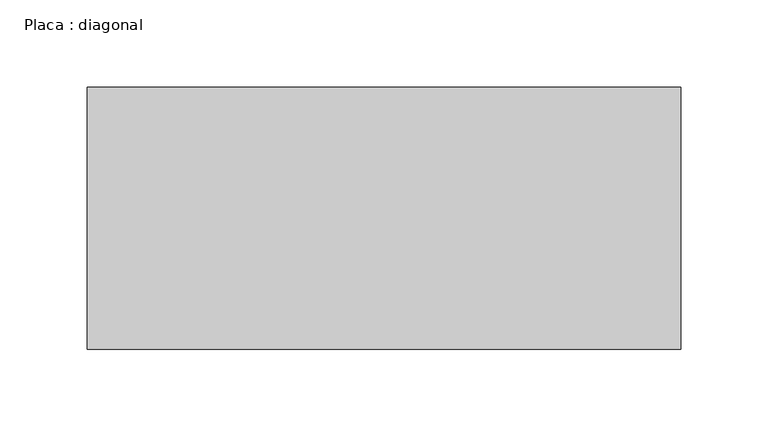
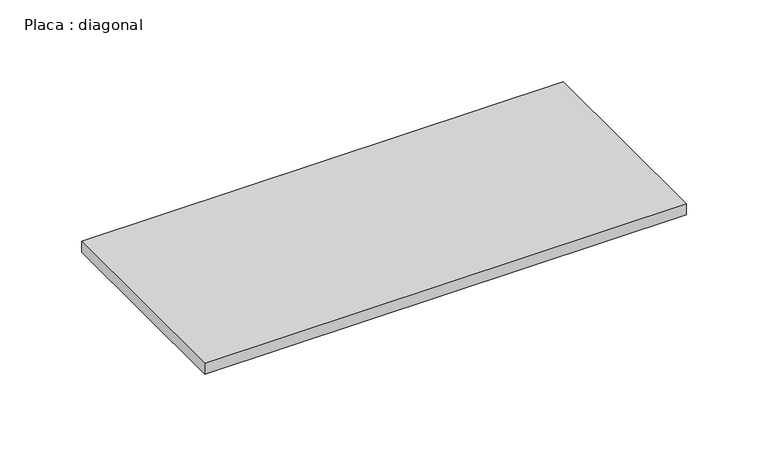
"""IFC4 building model written with IfcOpenShell, lengths in millimetres: beam geometry, Placa : diagonal."""

from ifc_helpers import new_model, si_unit, frame, origin, place, context, project, spatial, polyline, outline, extrude, source, transform, mapped, element, save


def placa_diagonal_9c3564dc(model_context):
    return source(origin(), model_context, "Body", "SweptSolid", [
        extrude(outline(polyline([(169.9719594, 75.0), (169.9719594, -75.0), (-169.5739247, -75.0), (-169.5739247, 75.0), (169.9719594, 75.0)])), frame((0.0, 0.0, -4.0), z_axis=(0.0, 0.0, 1.0), x_axis=(1.0, 0.0, 0.0)), (0.0, 0.0, 1.0), 8.0),
    ])


if __name__ == "__main__":
    model = new_model("IFC4")
    model_context = context("Model", 3, world=origin())
    ifc_project = project(units=[si_unit("LENGTHUNIT", "METRE", prefix="MILLI")], contexts=[model_context])
    site = spatial("IfcSite", under=ifc_project)
    building = spatial("IfcBuilding", under=site)
    placement = place(None, origin())
    placa_diagonal_shape = placa_diagonal_9c3564dc(model_context)
    element("IfcBeam", 1, ObjectType="Placa : diagonal", at=placement, inside=building, context=model_context, shape_type="MappedRepresentation", body=[
        mapped(placa_diagonal_shape, transform((0.0, 0.0, 0.0), x_axis=(1.0, 0.0, 0.0), y_axis=(0.0, 1.0, 0.0), z_axis=(0.0, 0.0, 1.0))),
    ])
    save(model, "model.ifc")

# Revit data of these elements
# Type "Placa : diagonal"
#   W = 0
#   Length [instance default] = 1.50 m
#   b = 0.15 m
#   d = 0.008 m
#   A = 0 m²
#   Structural Material [instance default] = Aço, 45-345
# Element 1 (IfcBeam, "Placa : diagonal")
#   Materials on its faces: "Aço, 45-345"
# Materials
#   "Aço, 45-345": class "Metal", colour RGB 247 247 247, transparency 0, Description = "Aço 345 MPa", Cost = 0
